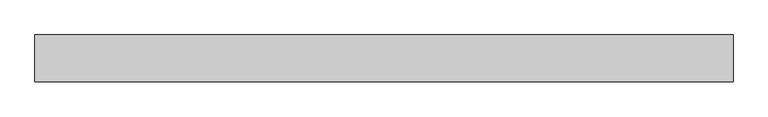
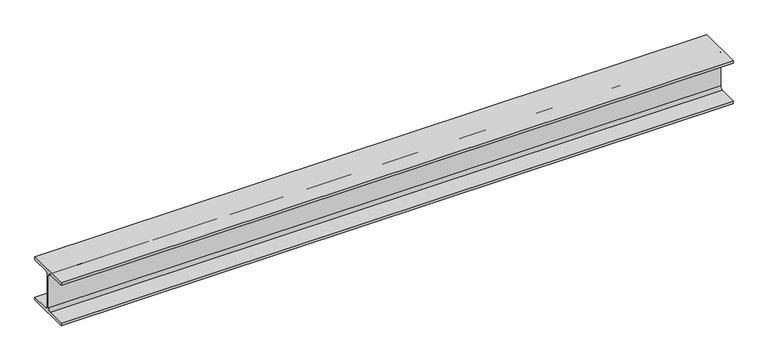
"""IFC4 building model written with IfcOpenShell, lengths in millimetres: beam geometry, 0912_Steel Framing_H-KSD3502 : H_SB_ASB_H-200x200x8x12."""

from ifc_helpers import new_model, si_unit, point, frame, frame_2d, origin, place, context, project, spatial, polyline, circle_curve, trimmed, segment, composite_curve, outline, extrude, source, transform, mapped, element, save


def beam_a5566726(model_context):
    return source(origin(), model_context, "Body", "SweptSolid", [
        extrude(outline(composite_curve([segment(polyline([(100.0, -88.0), (100.0, -100.0), (-100.0, -100.0), (-100.0, -88.0), (-17.0, -88.0)]), True, "CONTINUOUS"), segment(trimmed(circle_curve(frame_2d((-17.0, -75.0)), 13.0), [point((-17.0, -88.0))], [point((-4.0, -75.0))], True, "CARTESIAN"), True, "CONTINUOUS"), segment(polyline([(-4.0, -75.0), (-4.0, 75.0)]), True, "CONTINUOUS"), segment(trimmed(circle_curve(frame_2d((-17.0, 75.0)), 13.0), [point((-4.0, 75.0))], [point((-17.0, 88.0))], True, "CARTESIAN"), True, "CONTINUOUS"), segment(polyline([(-17.0, 88.0), (-100.0, 88.0), (-100.0, 100.0), (100.0, 100.0), (100.0, 88.0), (17.0, 88.0)]), True, "CONTINUOUS"), segment(trimmed(circle_curve(frame_2d((17.0, 75.0)), 13.0), [point((17.0, 88.0))], [point((4.0, 75.0))], True, "CARTESIAN"), True, "CONTINUOUS"), segment(polyline([(4.0, 75.0), (4.0, -75.0)]), True, "CONTINUOUS"), segment(trimmed(circle_curve(frame_2d((17.0, -75.0)), 13.0), [point((4.0, -75.0))], [point((17.0, -88.0))], True, "CARTESIAN"), True, "CONTINUOUS"), segment(polyline([(17.0, -88.0), (100.0, -88.0)]), True, "CONTINUOUS")], self_intersect=False)), frame((-1443.5851857, 0.0, 0.0), z_axis=(1.0, 0.0, 0.0), x_axis=(0.0, 1.0, 0.0)), (0.0, 0.0, 1.0), 2972.6935261),
    ])


if __name__ == "__main__":
    model = new_model("IFC4")
    model_context = context("Model", 3, world=origin())
    ifc_project = project(units=[si_unit("LENGTHUNIT", "METRE", prefix="MILLI")], contexts=[model_context])
    site = spatial("IfcSite", under=ifc_project)
    building = spatial("IfcBuilding", under=site)
    placement = place(None, origin())
    beam_shape = beam_a5566726(model_context)
    element("IfcBeam", 1, ObjectType="0912_Steel Framing_H-KSD3502 : H_SB_ASB_H-200x200x8x12", at=placement, inside=building, context=model_context, shape_type="MappedRepresentation", body=[
        mapped(beam_shape, transform((0.0, 0.0, 0.0), x_axis=(1.0, 0.0, 0.0), y_axis=(0.0, 1.0, 0.0), z_axis=(0.0, 0.0, 1.0))),
    ])
    save(model, "model.ifc")

# Revit data of these elements
# Type "0912_Steel Framing_H-KSD3502 : H_SB_ASB_H-200x200x8x12"
#   H_WM Code_1 = "S01AA002-00001 | Main Steel Structure Fabrication Work | Shelter/Building | Medium Steel - Standard (90KG/M>Weight≥30KG/M) | Material: (   )"
#   H_WM Code_2 = "S03AA028-00001 | Main Steel Structure Erection Work | Shelter/Building | Medium Steel (90KG/M>Weight≥30KG/M) | Material: (   )"
#   H_WM Code_3 = "S01AA010-00001 | Main Steel Structure Fabrication Work | Shelter/Building | Steel Painting/Coating | for Non-Fireproofed Steel Surface, Surface Preparation, Primer, Second & Final Coat | Material: (   )"
#   H_Q'ty Cal Type Tag = "SB-Q2"
#   Width = 20.0 cm
#   Web Thickness = 0.8 cm
#   Web Fillet = 1.3 cm
#   Warping Constant = 141000.0 cm⁶
#   W = 0
#   Torsional Moment of Inertia = 26.2485 cm⁴
#   Section Area = 63.53 cm²
#   Plastic Modulus weak axis = 244.0 cm³
#   Plastic Modulus strong axis = 525.0 cm³
#   Perimeter = 1.16 m²/m
#   Nominal Weight = 49.90 kgf/m
#   Moment of Inertia weak axis = 1600.00 cm⁴
#   Moment of Inertia strong axis = 4720.00 cm⁴
#   Height = 20.0 cm
#   Flange Thickness = 1.2 cm
#   Elastic Modulus weak axis = 160.0 cm³
#   Elastic Modulus strong axis = 472.0 cm³
#   Centroid Vertical = 10.0 cm
#   Centroid Horizontal = 10.0 cm
#   Ix = 47200000
#   Length [instance default] = 1.5240 m
#   Zx = 525000
#   b = 0.2000 m
#   h = 0.2000 m
#   r = 0.0130 m
#   s = 0.0080 m
#   t = 0.0120 m
#   A = 0.006353 m²
#   Structural Material [instance default] = Steel, 45-345
#   Assembly Code = ""
# Element 1 (IfcBeam, "0912_Steel Framing_H-KSD3502 : H_SB_ASB_H-200x200x8x12")
#   Structural Material = none
# Materials
#   "Steel, 45-345": class "Metal", colour RGB 189 187 185, transparency 0, Description = "Steel 345 MPa", Cost = 0
